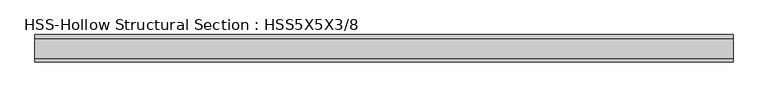
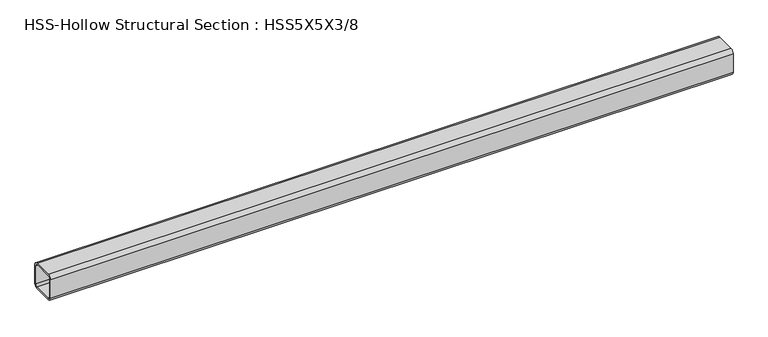
"""IFC4 building model written with IfcOpenShell, lengths in millimetres: member geometry, HSS-Hollow Structural Section : HSS5X5X3/8."""

from ifc_helpers import new_model, si_unit, point, frame, frame_2d, origin, place, context, project, spatial, polyline, circle_curve, trimmed, segment, composite_curve, outline, extrude, source, transform, mapped, element, save


def hss_hollow_structural_section_hss5x5x3_8_f21600e4(model_context):
    return source(origin(), model_context, "Body", "SweptSolid", [
        extrude(outline(composite_curve([segment(polyline([(63.5, 45.7708), (63.5, -45.7708)]), True, "CONTINUOUS"), segment(trimmed(circle_curve(frame_2d((45.7708, -45.7708)), 17.7292), [point((63.5, -45.7708))], [point((45.7708, -63.5))], False, "CARTESIAN"), True, "CONTINUOUS"), segment(polyline([(45.7708, -63.5), (-45.7708, -63.5)]), True, "CONTINUOUS"), segment(trimmed(circle_curve(frame_2d((-45.7708, -45.7708)), 17.7292), [point((-45.7708, -63.5))], [point((-63.5, -45.7708))], False, "CARTESIAN"), True, "CONTINUOUS"), segment(polyline([(-63.5, -45.7708), (-63.5, 45.7708)]), True, "CONTINUOUS"), segment(trimmed(circle_curve(frame_2d((-45.7708, 45.7708)), 17.7292), [point((-63.5, 45.7708))], [point((-45.7708, 63.5))], False, "CARTESIAN"), True, "CONTINUOUS"), segment(polyline([(-45.7708, 63.5), (45.7708, 63.5)]), True, "CONTINUOUS"), segment(trimmed(circle_curve(frame_2d((45.7708, 45.7708)), 17.7292), [point((45.7708, 63.5))], [point((63.5, 45.7708))], False, "CARTESIAN"), True, "CONTINUOUS")], self_intersect=False), holes=[composite_curve([segment(trimmed(circle_curve(frame_2d((-45.7708, 45.7708)), 8.8646), [point((-45.7708, 54.6354))], [point((-54.6354, 45.7708))], True, "CARTESIAN"), True, "CONTINUOUS"), segment(polyline([(-54.6354, 45.7708), (-54.6354, -45.7708)]), True, "CONTINUOUS"), segment(trimmed(circle_curve(frame_2d((-45.7708, -45.7708)), 8.8646), [point((-54.6354, -45.7708))], [point((-45.7708, -54.6354))], True, "CARTESIAN"), True, "CONTINUOUS"), segment(polyline([(-45.7708, -54.6354), (45.7708, -54.6354)]), True, "CONTINUOUS"), segment(trimmed(circle_curve(frame_2d((45.7708, -45.7708)), 8.8646), [point((45.7708, -54.6354))], [point((54.6354, -45.7708))], True, "CARTESIAN"), True, "CONTINUOUS"), segment(polyline([(54.6354, -45.7708), (54.6354, 45.7708)]), True, "CONTINUOUS"), segment(trimmed(circle_curve(frame_2d((45.7708, 45.7708)), 8.8646), [point((54.6354, 45.7708))], [point((45.7708, 54.6354))], True, "CARTESIAN"), True, "CONTINUOUS"), segment(polyline([(45.7708, 54.6354), (-45.7708, 54.6354)]), True, "CONTINUOUS")], self_intersect=False)]), frame((-1532.0508505, 0.0, 0.0), z_axis=(1.0, 0.0, 0.0), x_axis=(0.0, 1.0, 0.0)), (0.0, 0.0, 1.0), 3230.5088576),
    ])


if __name__ == "__main__":
    model = new_model("IFC4")
    model_context = context("Model", 3, world=origin())
    ifc_project = project(units=[si_unit("LENGTHUNIT", "METRE", prefix="MILLI")], contexts=[model_context])
    site = spatial("IfcSite", under=ifc_project)
    building = spatial("IfcBuilding", under=site)
    placement = place(None, origin())
    hss_hollow_structural_section_hss5x5x3_8_shape = hss_hollow_structural_section_hss5x5x3_8_f21600e4(model_context)
    element("IfcMember", 1, ObjectType="HSS-Hollow Structural Section : HSS5X5X3/8", at=placement, inside=building, context=model_context, shape_type="MappedRepresentation", body=[
        mapped(hss_hollow_structural_section_hss5x5x3_8_shape, transform((0.0, 0.0, 0.0), x_axis=(1.0, 0.0, 0.0), y_axis=(0.0, 1.0, 0.0), z_axis=(0.0, 0.0, 1.0))),
    ])
    save(model, "model.ifc")

# Revit data of these elements
# Type "HSS-Hollow Structural Section : HSS5X5X3/8"
#   Assembly Code = "B10"
#   Shape = "Square"
#   W = 22.3
#   Ht = 0' - 5"
#   Length [instance default] = 5' - 0"
#   b = 0' - 5"
#   kr = 0' - 0.698"
#   t = 0' - 0.349"
#   A = 0.0429167 SF
#   Structural Material [instance default] = Steel ASTM A500, Grade B, Rectangular and Square
# Element 1 (IfcMember, "HSS-Hollow Structural Section : HSS5X5X3/8")
#   Materials on its faces: "Steel ASTM A500, Grade B, Rectangular and Square"
# Materials
#   "Steel ASTM A500, Grade B, Rectangular and Square": class "Metal", colour RGB 199 199 199, transparency 0, Description = "Carbon steel", Cost = 0
